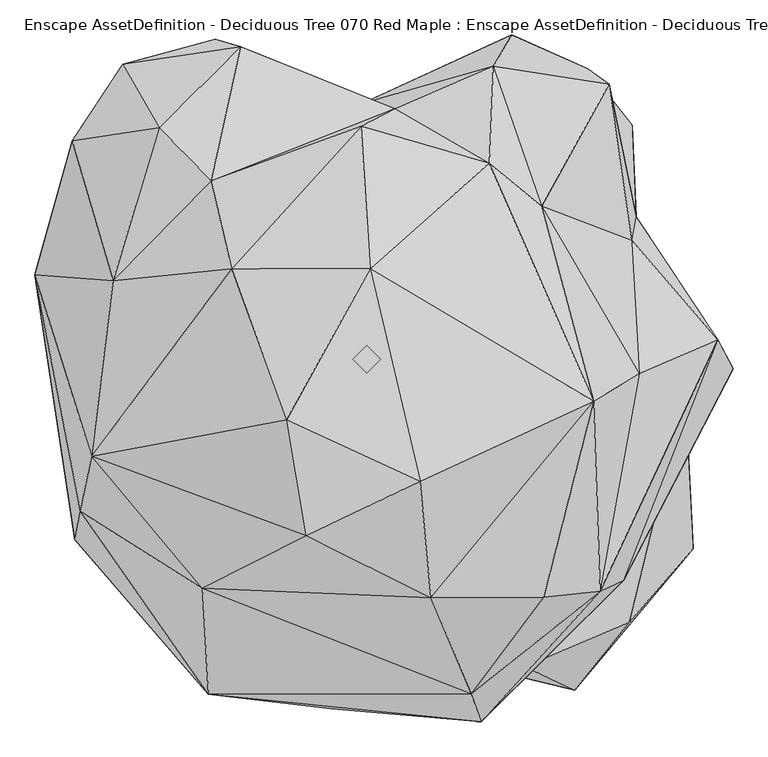
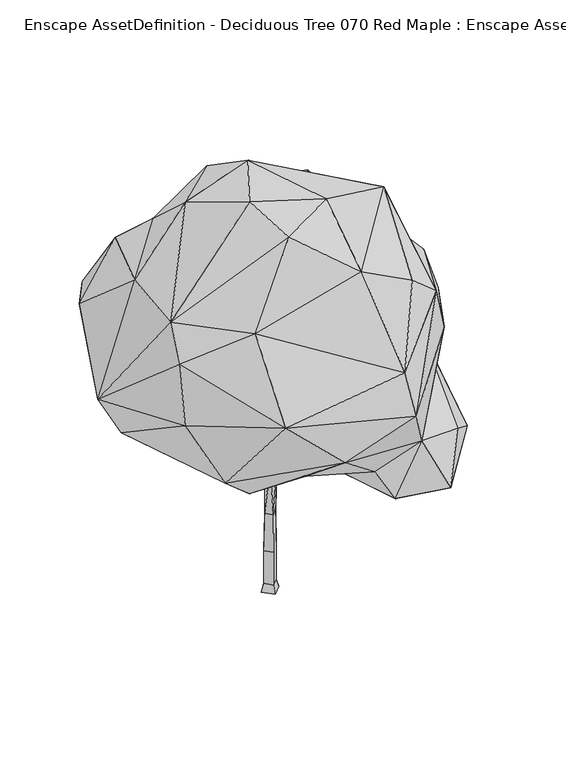
"""IFC4 building model written with IfcOpenShell, lengths in millimetres: geographic element geometry, Enscape AssetDefinition - Deciduous Tree 070 Red Maple : Enscape AssetDefinition - Deciduous Tree 070 Red Maple."""

from ifc_helpers import new_model, si_unit, origin, place, context, project, spatial, triangles, source, transform, mapped, element, save


def enscape_assetdefinition_deciduous_tree_070_red_maple_enscape_80613253(model_context):
    return source(origin(), model_context, "Body", "Tessellation", [
        triangles([(-0.005, -132.7059986, 174.1230018), (-132.7179982, -0.015, 174.9080011), (184.8849903, 0.0, 2.015), (0.0, -184.8849903, 2.0310001), (-133.3560044, -0.098, 904.5450056), (-184.8849903, 0.0, 2.5669999), (-0.09, 133.3079967, 909.3790129), (-0.019, 132.7159998, 175.7380013), (0.0, 184.8849903, 2.2), (133.359002, -0.163, 906.9989983), (81.2539975, -63.8019968, 1780.6770653), (57.8790026, -150.0210028, 2823.2730194), (-0.024, -133.3039999, 901.5459881), (-31.9520014, -177.2059895, 1776.492001), (-97.3330033, -170.8369924, 2831.8381943), (-145.4939989, -63.837001, 1780.9340263), (-103.9500049, 20.5839998, 2832.9459755), (-32.0179993, 49.378999, 1784.5019772), (89.6280049, 16.6640003, 2822.3820854), (39.1439997, -42.505, 3989.4660805), (112.7919979, -115.5359983, 3987.2040092), (-690.7539854, 462.0249962, 4187.1781403), (-33.9329987, -115.6969987, 3990.1910362), (39.2960026, -189.2500036, 3987.9318718), (855.4559961, 505.6160128, 4186.9839661), (619.0850315, -918.8439875, 4108.8858261), (-603.5440106, -935.4239347, 4105.7720627), (132.7220042, -0.028, 175.1649985), (2101.7871162, 2761.8488617, 5975.5922333), (2560.317849, 1356.6918983, 5370.2210449), (2523.1329094, 2226.7028927, 4380.2041489), (1716.340004, 2129.2200348, 3476.3787941), (1203.7970158, 2784.9611137, 6977.6118851), (1376.2479721, 3083.0711151, 4459.2789734), (698.9779747, 286.0999968, 3433.8610405), (2231.8210396, 445.3049775, 3706.3310371), (1299.3920528, -1115.0540314, 2886.3290543), (673.8889538, 2270.4250786, 3525.8432167), (300.0339937, 948.1060095, 3778.9870674), (-376.3430168, -690.3779909, 3543.3770302), (255.8279892, 352.5630003, 4090.191909), (-245.6800076, 1554.073019, 4262.8842751), (-1427.706023, 2146.5820564, 4417.6050636), (-1444.2659134, 790.005994, 3364.8059532), (-1342.2461231, -1291.9310257, 3480.2989037), (-2134.5040146, -2063.1840946, 4350.1548203), (-395.5039839, -1985.4529381, 3845.8309525), (240.5519958, -1027.9040457, 3486.8531548), (-1634.9580528, -2076.0960972, 3955.5300705), (-2773.4141441, -1714.6870525, 5644.7630081), (-1506.294976, -3183.7178787, 6030.996991), (-336.618007, -3323.3488907, 4939.1572403), (502.4279806, -2932.6788414, 4210.4839851), (953.6199898, -2896.0790405, 3436.4681488), (2166.8510227, -2325.356028, 2960.880899), (1978.4610683, -3142.9008934, 3468.7048439), (3102.893161, -1800.3510098, 3630.419973), (2699.3250618, -389.4630009, 3310.733091), (2493.9489349, -2499.0611229, 4213.7250664), (3026.941983, -304.3800038, 4780.5108192), (1500.7979279, -2922.3841209, 4537.7459862), (3481.98601, -87.351, 5528.1230347), (2442.4259171, -2097.9421474, 6237.7500687), (1085.9719402, -3444.886821, 5543.2976898), (3337.417218, 187.1080014, 6266.2640259), (2519.0479843, 1129.4080244, 6561.5018188), (2303.3749569, 2614.0529411, 6923.2832245), (2592.0670738, -138.7719983, 7171.5395828), (1663.8690788, 1454.8409946, 7672.7717789), (2156.3429432, -397.2930099, 8415.2851776), (2218.667046, -2204.3969868, 7181.4773483), (610.045031, -2265.1650799, 8209.9477112), (1680.1760777, -2262.4860283, 7641.0022064), (266.3159936, 2383.1309898, 6969.6623703), (1165.511998, 1862.9950058, 7854.2351212), (31.1890006, 859.4599669, 8993.5283707), (-53.4229973, 2214.6239788, 8078.9062912), (-1476.5809467, 1695.4340126, 7721.9711014), (-2410.5639084, 746.3960106, 7263.3636292), (-1196.2690596, 2970.4439781, 6571.3349396), (-37.9049992, 2435.0818886, 5037.6756454), (-1441.123954, 3042.7020676, 5598.8349976), (-2647.2369621, 825.9019861, 3898.8939926), (-2321.3269135, 2804.2111015, 5949.6333527), (-1974.2620514, 2200.4310951, 7165.5823883), (-2798.3788994, 2079.3399399, 6054.8170486), (-3154.2949654, 801.9150055, 4836.4611832), (-2615.9801491, -922.0650118, 7395.2549973), (-2723.0349518, -1443.9820644, 6823.2678177), (-758.3429558, -572.5580023, 9213.6364471), (-1562.1629322, -2177.4880188, 7533.8540955), (507.3990071, -1158.0009739, 9193.7504517), (-573.7689749, -1679.2618893, 9026.1211487), (-1285.350032, 862.8609947, 8513.004213), (992.8460112, -3179.253035, 6388.8989822)], [[95, 51, 64], [71, 73, 95], [71, 95, 64], [95, 73, 72], [76, 94, 90], [76, 90, 92], [72, 92, 93], [92, 90, 93], [91, 95, 72], [95, 91, 51], [72, 93, 91], [91, 89, 51], [89, 50, 51], [94, 88, 90], [91, 93, 88], [91, 88, 89], [88, 93, 90], [89, 88, 87], [50, 87, 83], [89, 87, 50], [88, 79, 87], [94, 79, 88], [79, 86, 87], [79, 85, 86], [87, 84, 83], [85, 84, 86], [86, 84, 87], [84, 43, 83], [84, 82, 43], [82, 81, 43], [80, 81, 82], [84, 80, 82], [80, 84, 85], [94, 78, 79], [80, 85, 78], [79, 78, 85], [94, 77, 78], [77, 94, 76], [74, 80, 78], [74, 78, 77], [74, 81, 80], [33, 81, 74], [75, 77, 76], [75, 33, 74], [75, 74, 77], [71, 70, 73], [70, 76, 92], [73, 70, 72], [72, 70, 92], [70, 75, 76], [71, 68, 70], [75, 70, 69], [68, 69, 70], [75, 69, 33], [69, 67, 33], [66, 69, 68], [66, 67, 69], [68, 65, 66], [68, 71, 65], [63, 64, 61], [63, 71, 64], [71, 63, 65], [65, 63, 62], [30, 66, 65], [67, 66, 30], [30, 65, 62], [62, 63, 60], [60, 63, 61], [60, 30, 62], [60, 61, 59], [59, 57, 60], [60, 57, 58], [57, 59, 56], [59, 61, 56], [57, 56, 55], [58, 57, 55], [37, 58, 55], [54, 56, 61], [55, 56, 54], [37, 55, 54], [54, 48, 37], [48, 54, 53], [61, 53, 54], [61, 52, 53], [52, 64, 51], [64, 52, 61], [51, 46, 52], [50, 46, 51], [50, 83, 46], [49, 52, 46], [47, 48, 53], [53, 52, 47], [47, 52, 49], [47, 49, 45], [83, 45, 46], [45, 49, 46], [40, 47, 45], [40, 48, 47], [44, 40, 45], [44, 45, 83], [43, 44, 83], [42, 44, 43], [81, 42, 43], [41, 48, 40], [42, 41, 44], [44, 41, 40], [42, 39, 41], [81, 38, 42], [42, 38, 39], [35, 41, 39], [41, 35, 48], [35, 39, 38], [48, 35, 37], [60, 58, 36], [35, 36, 37], [36, 58, 37], [30, 60, 36], [32, 36, 35], [32, 35, 38], [33, 34, 81], [34, 32, 38], [81, 34, 38], [32, 31, 36], [31, 30, 36], [34, 31, 32], [29, 31, 34], [33, 67, 29], [33, 29, 34], [29, 67, 30], [29, 30, 31], [9, 28, 3], [15, 26, 27], [15, 12, 26], [12, 25, 26], [12, 19, 25], [19, 22, 25], [19, 24, 12], [19, 21, 24], [12, 23, 15], [12, 24, 23], [15, 23, 20], [17, 27, 22], [17, 15, 27], [19, 17, 22], [15, 20, 17], [17, 21, 19], [17, 20, 21], [18, 17, 19], [16, 17, 18], [16, 15, 17], [5, 16, 18], [13, 16, 5], [14, 15, 16], [14, 12, 15], [13, 14, 16], [18, 19, 11], [11, 12, 14], [11, 19, 12], [10, 14, 13], [10, 11, 14], [28, 10, 13], [9, 8, 28], [6, 8, 9], [8, 10, 28], [5, 18, 7], [7, 11, 10], [7, 18, 11], [8, 7, 10], [4, 2, 6], [6, 2, 8], [2, 7, 8], [2, 5, 7], [4, 1, 2], [3, 1, 4], [3, 28, 1], [28, 13, 1], [1, 5, 2], [1, 13, 5]], closed=False),
    ])


if __name__ == "__main__":
    model = new_model("IFC4")
    model_context = context("Model", 3, world=origin())
    ifc_project = project(units=[si_unit("LENGTHUNIT", "METRE", prefix="MILLI")], contexts=[model_context])
    site = spatial("IfcSite", under=ifc_project)
    building = spatial("IfcBuilding", under=site)
    placement = place(None, origin())
    enscape_assetdefinition_deciduous_tree_070_red_maple_enscape_shape = enscape_assetdefinition_deciduous_tree_070_red_maple_enscape_80613253(model_context)
    element("IfcGeographicElement", 1, ObjectType="Enscape AssetDefinition - Deciduous Tree 070 Red Maple : Enscape AssetDefinition - Deciduous Tree 070 Red Maple", at=placement, inside=building, context=model_context, shape_type="MappedRepresentation", body=[
        mapped(enscape_assetdefinition_deciduous_tree_070_red_maple_enscape_shape, transform((0.0, 0.0, 0.0), x_axis=(1.0, 0.0, 0.0), y_axis=(0.0, 1.0, 0.0), z_axis=(0.0, 0.0, 1.0))),
    ])
    save(model, "model.ifc")

# Revit data of these elements
# Type "Enscape AssetDefinition - Deciduous Tree 070 Red Maple : Enscape AssetDefinition - Deciduous Tree 070 Red Maple"
#   EnscapeAssetSource = "REMOTE"
#   EnscapeAssetId = "9b9061d9-7e6b-454c-aee3-e29d52c98919"
#   Height = 9.213636 m
#   EnscapeNativeAssetHeight = 9.213636 m
#   Default Elevation = 0
